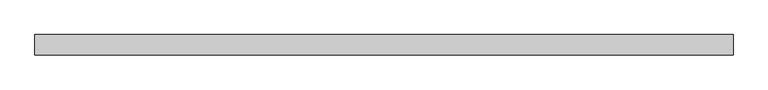
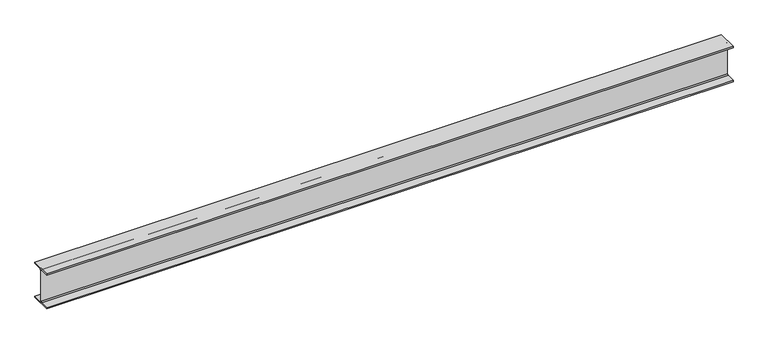
"""IFC4 building model written with IfcOpenShell, lengths in millimetres: beam geometry, Old_Steel Beam_H-KSD3502 : H_SB_ASB_H-200×200x8x12."""

from ifc_helpers import new_model, si_unit, point, frame, frame_2d, origin, place, context, project, spatial, polyline, circle_curve, trimmed, segment, composite_curve, outline, extrude, source, transform, mapped, element, save


def beam_c3a526f3(model_context):
    return source(origin(), model_context, "Body", "SweptSolid", [
        extrude(outline(composite_curve([segment(polyline([(82.5, -141.5), (82.5, -151.7), (-82.5, -151.7), (-82.5, -141.5), (-11.9, -141.5)]), True, "CONTINUOUS"), segment(trimmed(circle_curve(frame_2d((-11.9, -132.6)), 8.9), [point((-11.9, -141.5))], [point((-3.0, -132.6))], True, "CARTESIAN"), True, "CONTINUOUS"), segment(polyline([(-3.0, -132.6), (-3.0, 132.6)]), True, "CONTINUOUS"), segment(trimmed(circle_curve(frame_2d((-11.9, 132.6)), 8.9), [point((-3.0, 132.6))], [point((-11.9, 141.5))], True, "CARTESIAN"), True, "CONTINUOUS"), segment(polyline([(-11.9, 141.5), (-82.5, 141.5), (-82.5, 151.7), (82.5, 151.7), (82.5, 141.5), (11.9, 141.5)]), True, "CONTINUOUS"), segment(trimmed(circle_curve(frame_2d((11.9, 132.6)), 8.9), [point((11.9, 141.5))], [point((3.0, 132.6))], True, "CARTESIAN"), True, "CONTINUOUS"), segment(polyline([(3.0, 132.6), (3.0, -132.6)]), True, "CONTINUOUS"), segment(trimmed(circle_curve(frame_2d((11.9, -132.6)), 8.9), [point((3.0, -132.6))], [point((11.9, -141.5))], True, "CARTESIAN"), True, "CONTINUOUS"), segment(polyline([(11.9, -141.5), (82.5, -141.5)]), True, "CONTINUOUS")], self_intersect=False)), frame((-2793.5157367, 0.0, 0.0), z_axis=(1.0, 0.0, 0.0), x_axis=(0.0, 1.0, 0.0)), (0.0, 0.0, 1.0), 5619.4036777),
    ])


if __name__ == "__main__":
    model = new_model("IFC4")
    model_context = context("Model", 3, world=origin())
    ifc_project = project(units=[si_unit("LENGTHUNIT", "METRE", prefix="MILLI")], contexts=[model_context])
    site = spatial("IfcSite", under=ifc_project)
    building = spatial("IfcBuilding", under=site)
    placement = place(None, origin())
    beam_shape = beam_c3a526f3(model_context)
    element("IfcBeam", 1, ObjectType="Old_Steel Beam_H-KSD3502 : H_SB_ASB_H-200×200x8x12", at=placement, inside=building, context=model_context, shape_type="MappedRepresentation", body=[
        mapped(beam_shape, transform((0.0, 0.0, 0.0), x_axis=(1.0, 0.0, 0.0), y_axis=(0.0, 1.0, 0.0), z_axis=(0.0, 0.0, 1.0))),
    ])
    save(model, "model.ifc")

# Revit data of these elements
# Type "Old_Steel Beam_H-KSD3502 : H_SB_ASB_H-200×200x8x12"
#   Width = 20.0 cm
#   Web Thickness = 0.8 cm
#   Web Fillet = 1.3 cm
#   Warping Constant = 141376.0 cm⁶
#   Torsional Moment of Inertia = 26.2485 cm⁴
#   Torsional Modulus = 1.0 cm³
#   Section Area = 63.53 cm²
#   Plastic Modulus weak axis = 244.0 cm³
#   Plastic Modulus strong axis = 525.0 cm³
#   Perimeter = 1.16 m²/m
#   Nominal Weight = 49.90 kgf/m
#   Moment of Inertia weak axis = 1600.00 cm⁴
#   Moment of Inertia strong axis = 4720.00 cm⁴
#   Height = 20.0 cm
#   Flange Thickness = 1.2 cm
#   Elastic Modulus weak axis = 160.0 cm³
#   Elastic Modulus strong axis = 472.0 cm³
#   Centroid Vertical = 10.0 cm
#   Centroid Horizontal = 10.0 cm
#   Length [instance default] = 1.5240 m
#   Structural Material [instance default] = Steel, 45-345
#   Assembly Code = ""
# Element 1 (IfcBeam, "Old_Steel Beam_H-KSD3502 : H_SB_ASB_H-200×200x8x12")
#   Structural Material = none
# Materials
#   "Steel, 45-345": class "Metal", colour RGB 189 187 185, transparency 0, Description = "Steel 345 MPa", Cost = 0
